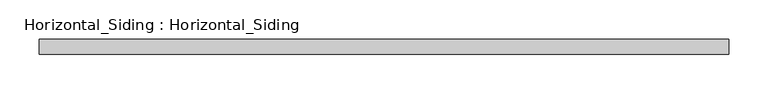
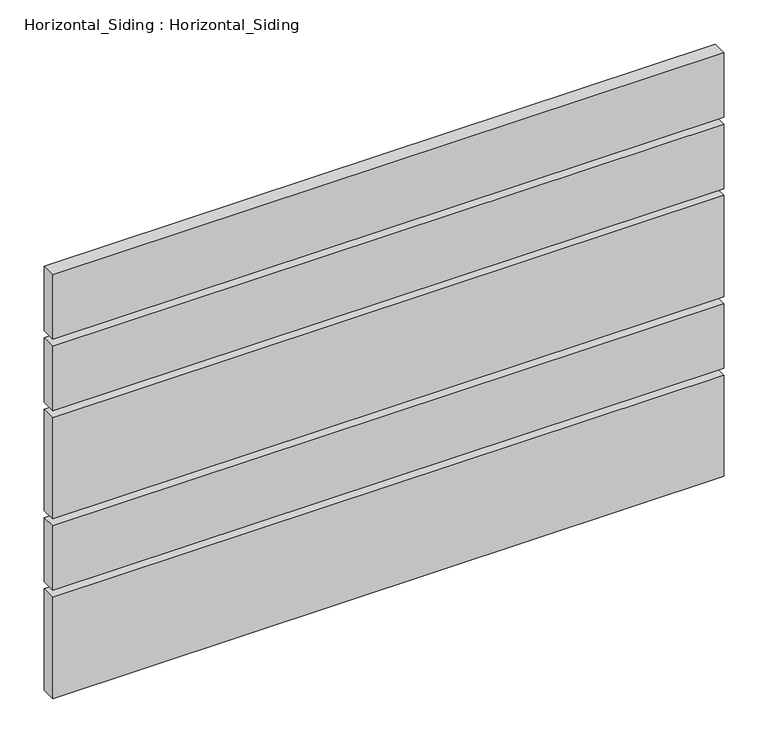
"""IFC4 building model written with IfcOpenShell, lengths in millimetres: plate geometry, Horizontal_Siding : Horizontal_Siding."""

from ifc_helpers import new_model, si_unit, frame, origin, place, context, project, spatial, polyline, outline, extrude, source, transform, mapped, element, save


def horizontal_siding_horizontal_siding_750e89fe(model_context):
    return source(origin(), model_context, "Body", "SweptSolid", [
        extrude(outline(polyline([(437.5115389, -19.05), (-437.5115389, -19.05), (-437.5115389, 0.0), (437.5115389, 0.0), (437.5115389, -19.05)])), frame((0.0, 0.0, 9.525), z_axis=(0.0, 0.0, 1.0), x_axis=(1.0, 0.0, 0.0)), (0.0, 0.0, 1.0), 139.7),
        extrude(outline(polyline([(437.5115389, -19.05), (-437.5115389, -19.05), (-437.5115389, 0.0), (437.5115389, 0.0), (437.5115389, -19.05)])), frame((0.0, 0.0, 158.75), z_axis=(0.0, 0.0, 1.0), x_axis=(1.0, 0.0, 0.0)), (0.0, 0.0, 1.0), 88.9),
        extrude(outline(polyline([(437.5115389, -19.05), (-437.5115389, -19.05), (-437.5115389, 0.0), (437.5115389, 0.0), (437.5115389, -19.05)])), frame((0.0, 0.0, 257.175), z_axis=(0.0, 0.0, 1.0), x_axis=(1.0, 0.0, 0.0)), (0.0, 0.0, 1.0), 139.7),
        extrude(outline(polyline([(437.5115389, -19.05), (-437.5115389, -19.05), (-437.5115389, 0.0), (437.5115389, 0.0), (437.5115389, -19.05)])), frame((0.0, 0.0, 406.4), z_axis=(0.0, 0.0, 1.0), x_axis=(1.0, 0.0, 0.0)), (0.0, 0.0, 1.0), 88.9),
        extrude(outline(polyline([(437.5115389, -19.05), (-437.5115389, -19.05), (-437.5115389, 0.0), (437.5115389, 0.0), (437.5115389, -19.05)])), frame((0.0, 0.0, 504.825), z_axis=(0.0, 0.0, 1.0), x_axis=(1.0, 0.0, 0.0)), (0.0, 0.0, 1.0), 88.9),
    ])


if __name__ == "__main__":
    model = new_model("IFC4")
    model_context = context("Model", 3, world=origin())
    ifc_project = project(units=[si_unit("LENGTHUNIT", "METRE", prefix="MILLI")], contexts=[model_context])
    site = spatial("IfcSite", under=ifc_project)
    building = spatial("IfcBuilding", under=site)
    placement = place(None, origin())
    horizontal_siding_horizontal_siding_shape = horizontal_siding_horizontal_siding_750e89fe(model_context)
    element("IfcPlate", 1, ObjectType="Horizontal_Siding : Horizontal_Siding", at=placement, inside=building, context=model_context, shape_type="MappedRepresentation", body=[
        mapped(horizontal_siding_horizontal_siding_shape, transform((0.0, 0.0, 0.0), x_axis=(1.0, 0.0, 0.0), y_axis=(0.0, 1.0, 0.0), z_axis=(0.0, 0.0, 1.0))),
    ])
    save(model, "model.ifc")

# Revit data of these elements
# Type "Horizontal_Siding : Horizontal_Siding"
#   Type Mark = "OUT"
#   Analytic Construction = "<None>"
#   extend = 0' - 2 3/4"
#   Width_2 = 0' - 3 1/2"
#   Width_1 = 0' - 5 1/2"
#   Gap = 0' - 0 3/8"
#   Plank Material = SLOTTED WOOD FENCE (THERMALLY MODIFIED WOOD: ARBOR WOOD)\n(EXTERIOR STAIN : PENOFIN VERDE EXT. STAIN - COLOR: CEDAR)
# Element 1 (IfcPlate, "Horizontal_Siding : Horizontal_Siding")
#   Materials on its faces: "SLOTTED WOOD FENCE (THERMALLY MODIFIED WOOD: ARBOR WOOD)\n(EXTERIOR STAIN : PENOFIN VERDE EXT. STAIN - COLOR: CEDAR)"
# Materials
#   "SLOTTED WOOD FENCE (THERMALLY MODIFIED WOOD: ARBOR WOOD)\n(EXTERIOR STAIN : PENOFIN VERDE EXT. STAIN - COLOR: CEDAR)": class "Wood", colour RGB 164 134 123, transparency 0, Description = "Pinus Echinata", Cost = 0
